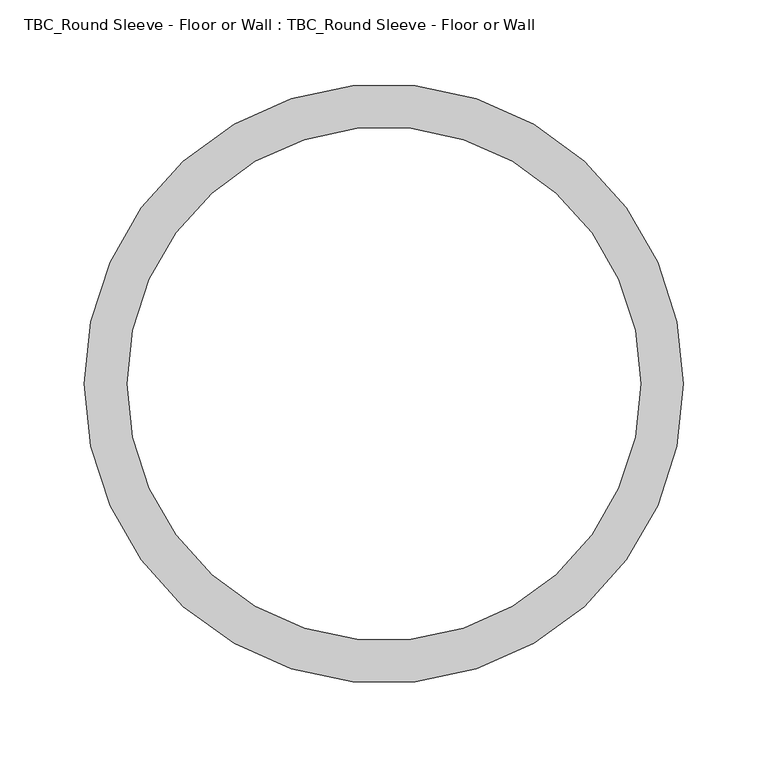
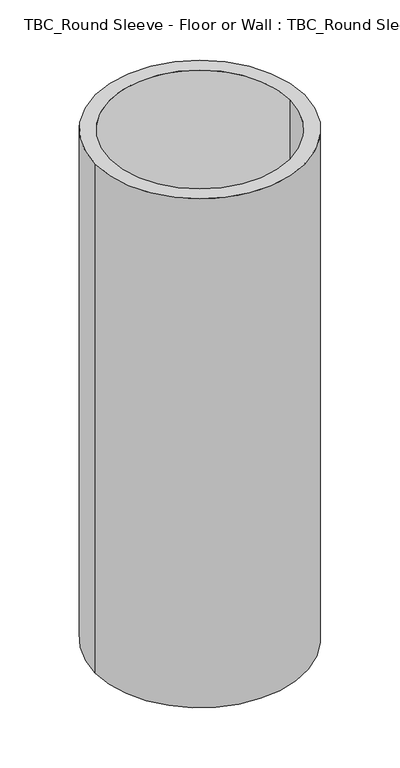
"""IFC4 building model written with IfcOpenShell, lengths in millimetres: proxy geometry, TBC_Round Sleeve - Floor or Wall : TBC_Round Sleeve - Floor or Wall."""

import ifcopenshell
import ifcopenshell.guid

model = None  # the IFC model being written
_history = None  # IfcOwnerHistory: only IFC2X3 demands one
_inside = {}  # id of a spatial element -> (the spatial element, [elements in it])
_under = {}  # id of a project, library or spatial element -> (it, [spatial elements below it])
_declared = {}  # id of a project -> (the project, [libraries it declares])
_typed = {}  # id of a type object -> (the type object, [elements of that type])
_made_of = {}  # id of a material, layer set ... -> (it, [elements and type objects made of it])


def new_model(schema):
    """Start an empty IFC model of exactly this schema.

    Asked for "IFC4X3", IfcOpenShell would pick the latest addendum, in which some entities
    have other attributes; the version numbers below select the first issue.
    IFC2X3 requires an IfcOwnerHistory on every rooted entity: one is made here for all.
    """
    global model, _history
    if schema == "IFC4X3":
        model = ifcopenshell.file(schema_version=(4, 3, 0, 0))
    else:
        model = ifcopenshell.file(schema=schema)
    _inside.clear()
    _under.clear()
    _declared.clear()
    _typed.clear()
    _made_of.clear()
    _history = None
    if model.schema == "IFC2X3":
        org = make("IfcOrganization", Name="unknown")
        user = make(
            "IfcPersonAndOrganization",
            ThePerson=make("IfcPerson", FamilyName="unknown"),
            TheOrganization=org,
        )
        app = make(
            "IfcApplication",
            ApplicationDeveloper=org,
            Version="unknown",
            ApplicationFullName="unknown",
            ApplicationIdentifier="unknown",
        )
        _history = make(
            "IfcOwnerHistory",
            OwningUser=user,
            OwningApplication=app,
            ChangeAction="ADDED",
            CreationDate=0,
        )
    return model


def make(cls, **values):
    """One entity of the class cls with the attributes given. An attribute that is None is left unset."""
    return model.create_entity(
        cls, **{name: value for name, value in values.items() if value is not None}
    )


def rooted(cls, **values):
    """An entity with a GlobalId (a new one), such as an element, a storey or a relation."""
    return make(cls, GlobalId=ifcopenshell.guid.new(), OwnerHistory=_history, **values)


def si_unit(unit_type, name, prefix=None):
    """IfcSIUnit, for example si_unit("LENGTHUNIT", "METRE", prefix="MILLI")."""
    return make("IfcSIUnit", UnitType=unit_type, Prefix=prefix, Name=name)


def assignment(units):
    """IfcUnitAssignment: the units of a project."""
    return None if units is None else make("IfcUnitAssignment", Units=units)


def point(xyz):
    """IfcCartesianPoint."""
    return None if xyz is None else make("IfcCartesianPoint", Coordinates=xyz)


def direction(xyz):
    """IfcDirection."""
    return None if xyz is None else make("IfcDirection", DirectionRatios=xyz)


def frame(location, z_axis=None, x_axis=None):
    """IfcAxis2Placement3D, a coordinate frame: its origin and axes. An axis left out is left unset."""
    return make(
        "IfcAxis2Placement3D",
        Location=point(location),
        Axis=direction(z_axis),
        RefDirection=direction(x_axis),
    )


def frame_2d(location, x_axis=None):
    """IfcAxis2Placement2D, a coordinate frame in the plane: its origin and x axis."""
    return make(
        "IfcAxis2Placement2D", Location=point(location), RefDirection=direction(x_axis)
    )


def origin():
    """The frame at (0, 0, 0) with its axes left unset."""
    return frame((0.0, 0.0, 0.0))


def origin_2d():
    """The frame at (0, 0) in the plane with its x axis left unset."""
    return frame_2d((0.0, 0.0))


def place(relative_to, where):
    """IfcLocalPlacement: puts the frame where relative to a parent placement (None: the world)."""
    return make(
        "IfcLocalPlacement", PlacementRelTo=relative_to, RelativePlacement=where
    )


def context(
    kind, dimensions, precision=None, world=None, true_north=None, identifier=None
):
    """IfcGeometricRepresentationContext, for example the 3D "Model" context."""
    return make(
        "IfcGeometricRepresentationContext",
        ContextIdentifier=identifier,
        ContextType=kind,
        CoordinateSpaceDimension=dimensions,
        Precision=precision,
        WorldCoordinateSystem=world,
        TrueNorth=true_north,
    )


def project(units=None, contexts=None):
    """IfcProject with its units and contexts."""
    return rooted(
        "IfcProject",
        Name="project",
        RepresentationContexts=contexts,
        UnitsInContext=assignment(units),
    )


def spatial(cls, under=None, at=None, **own):
    """A site, building, storey or space (cls), placed at a placement, below another one or the project."""
    s = rooted(cls, ObjectPlacement=at, **own)
    if under is not None:
        _under.setdefault(under.id(), (under, []))[1].append(s)
    return s


def circle_curve(where, radius):
    """IfcCircle in the frame where."""
    return make("IfcCircle", Position=where, Radius=radius)


def trimmed(basis, trim1, trim2, sense, master):
    """IfcTrimmedCurve: the piece of a basis curve between two trims."""
    return make(
        "IfcTrimmedCurve",
        BasisCurve=basis,
        Trim1=trim1,
        Trim2=trim2,
        SenseAgreement=sense,
        MasterRepresentation=master,
    )


def segment(curve, same_sense, transition):
    """IfcCompositeCurveSegment."""
    return make(
        "IfcCompositeCurveSegment",
        Transition=transition,
        SameSense=same_sense,
        ParentCurve=curve,
    )


def composite_curve(segments, self_intersect=None):
    """IfcCompositeCurve: segments joined end to end."""
    return make("IfcCompositeCurve", Segments=segments, SelfIntersect=self_intersect)


def outline(outer, holes=None, kind="AREA"):
    """IfcArbitraryClosedProfileDef: a profile drawn as a closed curve; with holes, ...WithVoids."""
    if holes is None:
        return make("IfcArbitraryClosedProfileDef", ProfileType=kind, OuterCurve=outer)
    return make(
        "IfcArbitraryProfileDefWithVoids",
        ProfileType=kind,
        OuterCurve=outer,
        InnerCurves=holes,
    )


def extrude(swept, where, along, depth):
    """IfcExtrudedAreaSolid: the profile swept, set in the frame where, extruded along a direction by depth."""
    return make(
        "IfcExtrudedAreaSolid",
        SweptArea=swept,
        Position=where,
        ExtrudedDirection=direction(along),
        Depth=depth,
    )


def shape(context_of_items, identifier, shape_type, items):
    """IfcShapeRepresentation: the items that make up one representation, for example the "Body"."""
    return make(
        "IfcShapeRepresentation",
        ContextOfItems=context_of_items,
        RepresentationIdentifier=identifier,
        RepresentationType=shape_type,
        Items=items,
    )


def source(mapping_origin, context_of_items, identifier, shape_type, items):
    """IfcRepresentationMap: a shape defined once, which mapped items show again and again."""
    return make(
        "IfcRepresentationMap",
        MappingOrigin=mapping_origin,
        MappedRepresentation=shape(context_of_items, identifier, shape_type, items),
    )


def transform(
    local_origin,
    x_axis=None,
    y_axis=None,
    z_axis=None,
    scale=None,
    scale2=None,
    scale3=None,
    uniform=True,
):
    """IfcCartesianTransformationOperator3D, or its non-uniform kind. x_axis, y_axis, z_axis: its Axis1, 2, 3."""
    if uniform:
        return make(
            "IfcCartesianTransformationOperator3D",
            Axis1=direction(x_axis),
            Axis2=direction(y_axis),
            LocalOrigin=point(local_origin),
            Scale=scale,
            Axis3=direction(z_axis),
        )
    return make(
        "IfcCartesianTransformationOperator3DnonUniform",
        Axis1=direction(x_axis),
        Axis2=direction(y_axis),
        LocalOrigin=point(local_origin),
        Scale=scale,
        Axis3=direction(z_axis),
        Scale2=scale2,
        Scale3=scale3,
    )


def mapped(mapping_source, mapping_target):
    """IfcMappedItem: shows the shape of a source again, moved by a transform."""
    return make(
        "IfcMappedItem", MappingSource=mapping_source, MappingTarget=mapping_target
    )


def made_of(thing, what):
    """Note that an element or type object is made of a material, layer set ...; save() writes the relation."""
    if what is not None:
        _made_of.setdefault(what.id(), (what, []))[1].append(thing)
    return thing


def element(
    cls,
    number,
    at=None,
    inside=None,
    cuts=None,
    type_object=None,
    material=None,
    context=None,
    identifier="Body",
    shape_type=None,
    held_by="IfcProductDefinitionShape",
    body=None,
    shapes=None,
    **own,
):
    """One element of the class cls, such as IfcWall. Its Tag is "e" and its number.

    at: its placement. inside: the storey or other place that contains it. cuts: it is an
    opening in that element (IfcRelVoidsElement). A single representation is given by context,
    identifier, shape_type and body (its items); several are given by shapes. held_by: the class
    of the entity that holds the representations. save() writes the other relations.
    """
    e = rooted(cls, Tag="e%d" % number, ObjectPlacement=at, **own)
    if body is not None:
        shapes = [shape(context, identifier, shape_type, body)]
    if shapes is not None:
        e.Representation = make(held_by, Representations=shapes)
    if inside is not None:
        _inside.setdefault(inside.id(), (inside, []))[1].append(e)
    if cuts is not None:
        rooted(
            "IfcRelVoidsElement", RelatingBuildingElement=cuts, RelatedOpeningElement=e
        )
    if type_object is not None:
        _typed.setdefault(type_object.id(), (type_object, []))[1].append(e)
    return made_of(e, material)


def aggregate(whole, parts):
    """IfcRelAggregates: a whole, such as a stair, and the parts it consists of."""
    return rooted("IfcRelAggregates", RelatingObject=whole, RelatedObjects=parts)


def save(model, path):
    """Write the relations noted so far, then the file.

    IfcRelAggregates (storeys below a building ...), IfcRelContainedInSpatialStructure (elements
    in a storey), IfcRelDefinesByType, IfcRelAssociatesMaterial and IfcRelDeclares: one each for
    every whole, place, type object, material and project.
    """
    for whole, parts in _under.values():
        aggregate(whole, parts)
    for where, things in _inside.values():
        rooted(
            "IfcRelContainedInSpatialStructure",
            RelatedElements=things,
            RelatingStructure=where,
        )
    for kind, things in _typed.values():
        rooted("IfcRelDefinesByType", RelatedObjects=things, RelatingType=kind)
    for what, things in _made_of.values():
        rooted("IfcRelAssociatesMaterial", RelatedObjects=things, RelatingMaterial=what)
    for by, libraries in _declared.values():
        rooted("IfcRelDeclares", RelatingContext=by, RelatedDefinitions=libraries)
    model.write(path)


def tbc_round_sleeve_floor_or_wall_tbc_round_sleeve_floor_or_7fc3faad(model_context):
    return source(origin(), model_context, "Body", "SweptSolid", [
        extrude(outline(composite_curve([segment(trimmed(circle_curve(origin_2d(), 177.8), [point((-177.8, 0.0))], [point((177.8, 0.0))], False, "CARTESIAN"), True, "CONTINUOUS"), segment(trimmed(circle_curve(origin_2d(), 177.8), [point((177.8, 0.0))], [point((-177.8, 0.0))], False, "CARTESIAN"), True, "CONTINUOUS")], self_intersect=False), holes=[composite_curve([segment(trimmed(circle_curve(origin_2d(), 152.4), [point((-152.4, 0.0))], [point((152.4, 0.0))], True, "CARTESIAN"), True, "CONTINUOUS"), segment(trimmed(circle_curve(origin_2d(), 152.4), [point((152.4, 0.0))], [point((-152.4, 0.0))], True, "CARTESIAN"), True, "CONTINUOUS")], self_intersect=False)]), frame((0.0, 0.0, -914.4), z_axis=(0.0, 0.0, 1.0), x_axis=(1.0, 0.0, 0.0)), (0.0, 0.0, 1.0), 914.4),
    ])


if __name__ == "__main__":
    model = new_model("IFC4")
    model_context = context("Model", 3, world=origin())
    ifc_project = project(units=[si_unit("LENGTHUNIT", "METRE", prefix="MILLI")], contexts=[model_context])
    site = spatial("IfcSite", under=ifc_project)
    building = spatial("IfcBuilding", under=site)
    placement = place(None, origin())
    tbc_round_sleeve_floor_or_wall_tbc_round_sleeve_floor_or_shape = tbc_round_sleeve_floor_or_wall_tbc_round_sleeve_floor_or_7fc3faad(model_context)
    element("IfcBuildingElementProxy", 1, Name="TBC_Round Sleeve - Floor or Wall : TBC_Round Sleeve - Floor or Wall", ObjectType="TBC_Round Sleeve - Floor or Wall : TBC_Round Sleeve - Floor or Wall", at=placement, inside=building, context=model_context, shape_type="MappedRepresentation", body=[
        mapped(tbc_round_sleeve_floor_or_wall_tbc_round_sleeve_floor_or_shape, transform((0.0, 0.0, 0.0), x_axis=(1.0, 0.0, 0.0), y_axis=(0.0, 1.0, 0.0), z_axis=(0.0, 0.0, 1.0))),
    ])
    save(model, "model.ifc")

# Revit data of these elements
# Project information
#   Project Issue Date = "Issue Date"
#   Project Status = "Project Status"
#   Client Name = "Owner"
#   Project Address = "Enter address here"
#   Project Name = "Project Name"
#   Project Number = "Project Number"
# Type "TBC_Round Sleeve - Floor or Wall : TBC_Round Sleeve - Floor or Wall"
#   Tag Dimension [instance default] = ""
#   MEP Type [instance default] = ""
#   MEP Element [instance default] = ""
#   MEP Category [instance default] = ""
#   Host Element Type [instance default] = ""
#   Host Element Id [instance default] = ""
#   Host Element Category [instance default] = ""
#   Control Line Y [instance default] = ""
#   Control Line X [instance default] = ""
#   Sleeve Radius [instance default] = 1' - 0"
#   Sleeve Edge [instance default] = 1' - 2"
#   Sleeve Depth [instance default] = 3' - 0"
#   Distance Y [instance default] = 0' - 0"
#   Distance X [instance default] = 0' - 0"
#   Default Elevation = 0
